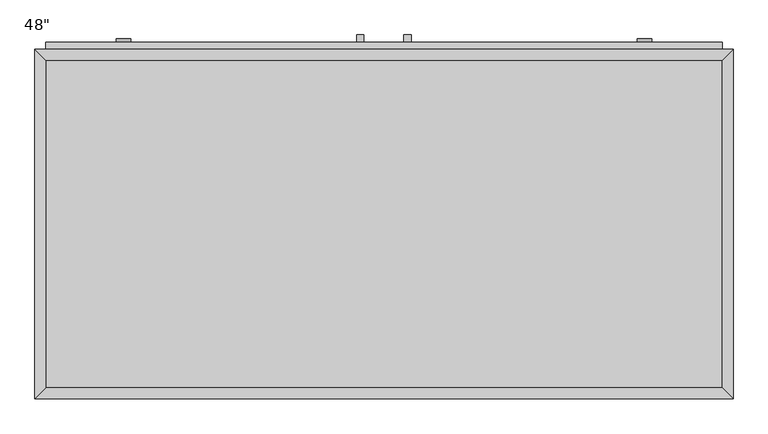
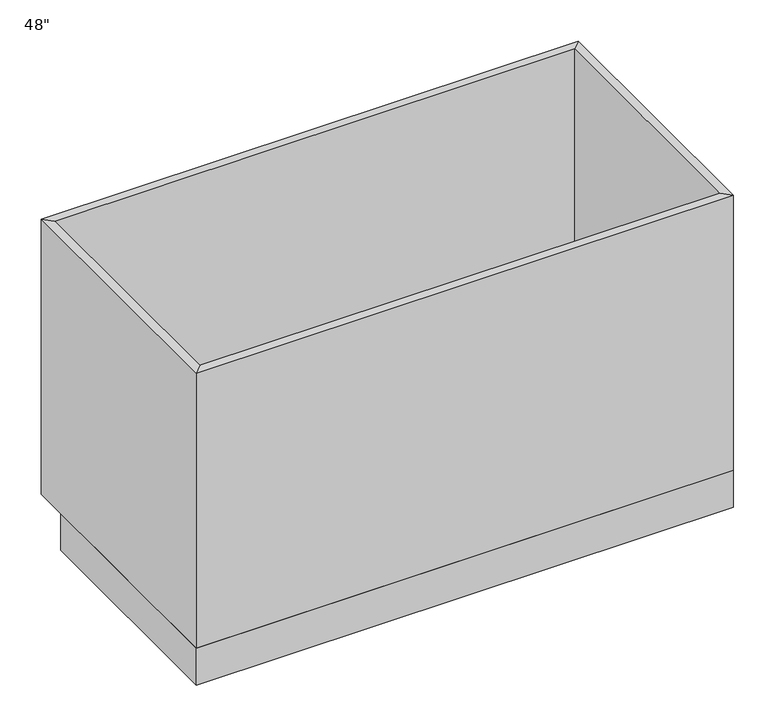
"""IFC4 building model written with IfcOpenShell, lengths in millimetres: furniture geometry."""

import ifcopenshell
import ifcopenshell.guid

model = None  # the IFC model being written
_history = None  # IfcOwnerHistory: only IFC2X3 demands one
_inside = {}  # id of a spatial element -> (the spatial element, [elements in it])
_under = {}  # id of a project, library or spatial element -> (it, [spatial elements below it])
_declared = {}  # id of a project -> (the project, [libraries it declares])
_typed = {}  # id of a type object -> (the type object, [elements of that type])
_made_of = {}  # id of a material, layer set ... -> (it, [elements and type objects made of it])


def new_model(schema):
    """Start an empty IFC model of exactly this schema.

    Asked for "IFC4X3", IfcOpenShell would pick the latest addendum, in which some entities
    have other attributes; the version numbers below select the first issue.
    IFC2X3 requires an IfcOwnerHistory on every rooted entity: one is made here for all.
    """
    global model, _history
    if schema == "IFC4X3":
        model = ifcopenshell.file(schema_version=(4, 3, 0, 0))
    else:
        model = ifcopenshell.file(schema=schema)
    _inside.clear()
    _under.clear()
    _declared.clear()
    _typed.clear()
    _made_of.clear()
    _history = None
    if model.schema == "IFC2X3":
        org = make("IfcOrganization", Name="unknown")
        user = make(
            "IfcPersonAndOrganization",
            ThePerson=make("IfcPerson", FamilyName="unknown"),
            TheOrganization=org,
        )
        app = make(
            "IfcApplication",
            ApplicationDeveloper=org,
            Version="unknown",
            ApplicationFullName="unknown",
            ApplicationIdentifier="unknown",
        )
        _history = make(
            "IfcOwnerHistory",
            OwningUser=user,
            OwningApplication=app,
            ChangeAction="ADDED",
            CreationDate=0,
        )
    return model


def make(cls, **values):
    """One entity of the class cls with the attributes given. An attribute that is None is left unset."""
    return model.create_entity(
        cls, **{name: value for name, value in values.items() if value is not None}
    )


def rooted(cls, **values):
    """An entity with a GlobalId (a new one), such as an element, a storey or a relation."""
    return make(cls, GlobalId=ifcopenshell.guid.new(), OwnerHistory=_history, **values)


def si_unit(unit_type, name, prefix=None):
    """IfcSIUnit, for example si_unit("LENGTHUNIT", "METRE", prefix="MILLI")."""
    return make("IfcSIUnit", UnitType=unit_type, Prefix=prefix, Name=name)


def assignment(units):
    """IfcUnitAssignment: the units of a project."""
    return None if units is None else make("IfcUnitAssignment", Units=units)


def point(xyz):
    """IfcCartesianPoint."""
    return None if xyz is None else make("IfcCartesianPoint", Coordinates=xyz)


def direction(xyz):
    """IfcDirection."""
    return None if xyz is None else make("IfcDirection", DirectionRatios=xyz)


def frame(location, z_axis=None, x_axis=None):
    """IfcAxis2Placement3D, a coordinate frame: its origin and axes. An axis left out is left unset."""
    return make(
        "IfcAxis2Placement3D",
        Location=point(location),
        Axis=direction(z_axis),
        RefDirection=direction(x_axis),
    )


def frame_2d(location, x_axis=None):
    """IfcAxis2Placement2D, a coordinate frame in the plane: its origin and x axis."""
    return make(
        "IfcAxis2Placement2D", Location=point(location), RefDirection=direction(x_axis)
    )


def origin():
    """The frame at (0, 0, 0) with its axes left unset."""
    return frame((0.0, 0.0, 0.0))


def origin_with_axes():
    """The frame at (0, 0, 0) with the z axis (0, 0, 1) and the x axis (1, 0, 0) written out."""
    return frame((0.0, 0.0, 0.0), z_axis=(0.0, 0.0, 1.0), x_axis=(1.0, 0.0, 0.0))


def place(relative_to, where):
    """IfcLocalPlacement: puts the frame where relative to a parent placement (None: the world)."""
    return make(
        "IfcLocalPlacement", PlacementRelTo=relative_to, RelativePlacement=where
    )


def context(
    kind, dimensions, precision=None, world=None, true_north=None, identifier=None
):
    """IfcGeometricRepresentationContext, for example the 3D "Model" context."""
    return make(
        "IfcGeometricRepresentationContext",
        ContextIdentifier=identifier,
        ContextType=kind,
        CoordinateSpaceDimension=dimensions,
        Precision=precision,
        WorldCoordinateSystem=world,
        TrueNorth=true_north,
    )


def project(units=None, contexts=None):
    """IfcProject with its units and contexts."""
    return rooted(
        "IfcProject",
        Name="project",
        RepresentationContexts=contexts,
        UnitsInContext=assignment(units),
    )


def spatial(cls, under=None, at=None, **own):
    """A site, building, storey or space (cls), placed at a placement, below another one or the project."""
    s = rooted(cls, ObjectPlacement=at, **own)
    if under is not None:
        _under.setdefault(under.id(), (under, []))[1].append(s)
    return s


def polyline(points):
    """IfcPolyline through the points."""
    return make("IfcPolyline", Points=[point(p) for p in points])


def circle_curve(where, radius):
    """IfcCircle in the frame where."""
    return make("IfcCircle", Position=where, Radius=radius)


def trimmed(basis, trim1, trim2, sense, master):
    """IfcTrimmedCurve: the piece of a basis curve between two trims."""
    return make(
        "IfcTrimmedCurve",
        BasisCurve=basis,
        Trim1=trim1,
        Trim2=trim2,
        SenseAgreement=sense,
        MasterRepresentation=master,
    )


def segment(curve, same_sense, transition):
    """IfcCompositeCurveSegment."""
    return make(
        "IfcCompositeCurveSegment",
        Transition=transition,
        SameSense=same_sense,
        ParentCurve=curve,
    )


def composite_curve(segments, self_intersect=None):
    """IfcCompositeCurve: segments joined end to end."""
    return make("IfcCompositeCurve", Segments=segments, SelfIntersect=self_intersect)


def outline(outer, holes=None, kind="AREA"):
    """IfcArbitraryClosedProfileDef: a profile drawn as a closed curve; with holes, ...WithVoids."""
    if holes is None:
        return make("IfcArbitraryClosedProfileDef", ProfileType=kind, OuterCurve=outer)
    return make(
        "IfcArbitraryProfileDefWithVoids",
        ProfileType=kind,
        OuterCurve=outer,
        InnerCurves=holes,
    )


def extrude(swept, where, along, depth):
    """IfcExtrudedAreaSolid: the profile swept, set in the frame where, extruded along a direction by depth."""
    return make(
        "IfcExtrudedAreaSolid",
        SweptArea=swept,
        Position=where,
        ExtrudedDirection=direction(along),
        Depth=depth,
    )


def faces_of(points, faces, orient=None, outer=None):
    """IfcFace entities. A face is a list of loops; a loop is a list of indices into points, from 0.

    orient and outer hold one flag for each loop. By default every Orientation is true, the
    first loop of a face is its IfcFaceOuterBound and the others are IfcFaceBound.
    """
    made = []
    for i, loops in enumerate(faces):
        bounds = []
        for j, loop in enumerate(loops):
            is_outer = j == 0 if outer is None else outer[i][j]
            bounds.append(
                make(
                    "IfcFaceOuterBound" if is_outer else "IfcFaceBound",
                    Bound=make("IfcPolyLoop", Polygon=[points[k] for k in loop]),
                    Orientation=True if orient is None else orient[i][j],
                )
            )
        made.append(make("IfcFace", Bounds=bounds))
    return made


def faceted_brep(points, faces, orient=None, outer=None, voids=None):
    """IfcFacetedBrep: a solid bounded by flat faces; with voids (closed shells), ...WithVoids."""
    shared = [point(p) for p in points]
    hull = make("IfcClosedShell", CfsFaces=faces_of(shared, faces, orient, outer))
    if voids is None:
        return make("IfcFacetedBrep", Outer=hull)
    return make(
        "IfcFacetedBrepWithVoids",
        Outer=hull,
        Voids=[
            make(cls, CfsFaces=faces_of(shared, fs, o, b)) for cls, fs, o, b in voids
        ],
    )


def shape(context_of_items, identifier, shape_type, items):
    """IfcShapeRepresentation: the items that make up one representation, for example the "Body"."""
    return make(
        "IfcShapeRepresentation",
        ContextOfItems=context_of_items,
        RepresentationIdentifier=identifier,
        RepresentationType=shape_type,
        Items=items,
    )


def source(mapping_origin, context_of_items, identifier, shape_type, items):
    """IfcRepresentationMap: a shape defined once, which mapped items show again and again."""
    return make(
        "IfcRepresentationMap",
        MappingOrigin=mapping_origin,
        MappedRepresentation=shape(context_of_items, identifier, shape_type, items),
    )


def transform(
    local_origin,
    x_axis=None,
    y_axis=None,
    z_axis=None,
    scale=None,
    scale2=None,
    scale3=None,
    uniform=True,
):
    """IfcCartesianTransformationOperator3D, or its non-uniform kind. x_axis, y_axis, z_axis: its Axis1, 2, 3."""
    if uniform:
        return make(
            "IfcCartesianTransformationOperator3D",
            Axis1=direction(x_axis),
            Axis2=direction(y_axis),
            LocalOrigin=point(local_origin),
            Scale=scale,
            Axis3=direction(z_axis),
        )
    return make(
        "IfcCartesianTransformationOperator3DnonUniform",
        Axis1=direction(x_axis),
        Axis2=direction(y_axis),
        LocalOrigin=point(local_origin),
        Scale=scale,
        Axis3=direction(z_axis),
        Scale2=scale2,
        Scale3=scale3,
    )


def mapped(mapping_source, mapping_target):
    """IfcMappedItem: shows the shape of a source again, moved by a transform."""
    return make(
        "IfcMappedItem", MappingSource=mapping_source, MappingTarget=mapping_target
    )


def made_of(thing, what):
    """Note that an element or type object is made of a material, layer set ...; save() writes the relation."""
    if what is not None:
        _made_of.setdefault(what.id(), (what, []))[1].append(thing)
    return thing


def element(
    cls,
    number,
    at=None,
    inside=None,
    cuts=None,
    type_object=None,
    material=None,
    context=None,
    identifier="Body",
    shape_type=None,
    held_by="IfcProductDefinitionShape",
    body=None,
    shapes=None,
    **own,
):
    """One element of the class cls, such as IfcWall. Its Tag is "e" and its number.

    at: its placement. inside: the storey or other place that contains it. cuts: it is an
    opening in that element (IfcRelVoidsElement). A single representation is given by context,
    identifier, shape_type and body (its items); several are given by shapes. held_by: the class
    of the entity that holds the representations. save() writes the other relations.
    """
    e = rooted(cls, Tag="e%d" % number, ObjectPlacement=at, **own)
    if body is not None:
        shapes = [shape(context, identifier, shape_type, body)]
    if shapes is not None:
        e.Representation = make(held_by, Representations=shapes)
    if inside is not None:
        _inside.setdefault(inside.id(), (inside, []))[1].append(e)
    if cuts is not None:
        rooted(
            "IfcRelVoidsElement", RelatingBuildingElement=cuts, RelatedOpeningElement=e
        )
    if type_object is not None:
        _typed.setdefault(type_object.id(), (type_object, []))[1].append(e)
    return made_of(e, material)


def aggregate(whole, parts):
    """IfcRelAggregates: a whole, such as a stair, and the parts it consists of."""
    return rooted("IfcRelAggregates", RelatingObject=whole, RelatedObjects=parts)


def save(model, path):
    """Write the relations noted so far, then the file.

    IfcRelAggregates (storeys below a building ...), IfcRelContainedInSpatialStructure (elements
    in a storey), IfcRelDefinesByType, IfcRelAssociatesMaterial and IfcRelDeclares: one each for
    every whole, place, type object, material and project.
    """
    for whole, parts in _under.values():
        aggregate(whole, parts)
    for where, things in _inside.values():
        rooted(
            "IfcRelContainedInSpatialStructure",
            RelatedElements=things,
            RelatingStructure=where,
        )
    for kind, things in _typed.values():
        rooted("IfcRelDefinesByType", RelatedObjects=things, RelatingType=kind)
    for what, things in _made_of.values():
        rooted("IfcRelAssociatesMaterial", RelatedObjects=things, RelatingMaterial=what)
    for by, libraries in _declared.values():
        rooted("IfcRelDeclares", RelatingContext=by, RelatedDefinitions=libraries)
    model.write(path)


def furniture_1910af95(model_context):
    return source(origin(), model_context, "Body", "SolidModel", [
        extrude(outline(polyline([(55.91996, 635.0), (55.91996, 622.3), (43.21996, 622.3), (43.21996, 635.0), (55.91996, 635.0)])), frame((0.0, 0.0, 469.9), z_axis=(0.0, 0.0, 1.0), x_axis=(1.0, 0.0, 0.0)), (0.0, 0.0, 1.0), 101.6),
        extrude(outline(polyline([(138.46996, 635.0), (138.46996, 622.3), (125.76996, 622.3), (125.76996, 635.0), (138.46996, 635.0)])), frame((0.0, 0.0, 469.9), z_axis=(0.0, 0.0, 1.0), x_axis=(1.0, 0.0, 0.0)), (0.0, 0.0, 1.0), 101.6),
        extrude(outline(composite_curve([segment(trimmed(circle_curve(frame_2d((484.1875, -363.97379)), 12.7), [point((484.1875, -376.67379))], [point((484.1875, -351.27379))], False, "CARTESIAN"), True, "CONTINUOUS"), segment(trimmed(circle_curve(frame_2d((484.1875, -363.97379)), 12.7), [point((484.1875, -351.27379))], [point((484.1875, -376.67379))], False, "CARTESIAN"), True, "CONTINUOUS")], self_intersect=False)), frame((0.0, 622.3, 0.0), z_axis=(0.0, 1.0, 0.0), x_axis=(0.0, 0.0, 1.0)), (0.0, 0.0, 1.0), 6.35),
        extrude(outline(composite_curve([segment(trimmed(circle_curve(frame_2d((233.3625, -363.97379)), 12.7), [point((233.3625, -376.67379))], [point((233.3625, -351.27379))], False, "CARTESIAN"), True, "CONTINUOUS"), segment(trimmed(circle_curve(frame_2d((233.3625, -363.97379)), 12.7), [point((233.3625, -351.27379))], [point((233.3625, -376.67379))], False, "CARTESIAN"), True, "CONTINUOUS")], self_intersect=False)), frame((0.0, 622.3, 0.0), z_axis=(0.0, 1.0, 0.0), x_axis=(0.0, 0.0, 1.0)), (0.0, 0.0, 1.0), 6.35),
        extrude(outline(composite_curve([segment(trimmed(circle_curve(frame_2d((233.3625, 545.66371)), 12.7), [point((233.3625, 532.96371))], [point((233.3625, 558.36371))], False, "CARTESIAN"), True, "CONTINUOUS"), segment(trimmed(circle_curve(frame_2d((233.3625, 545.66371)), 12.7), [point((233.3625, 558.36371))], [point((233.3625, 532.96371))], False, "CARTESIAN"), True, "CONTINUOUS")], self_intersect=False)), frame((0.0, 622.3, 0.0), z_axis=(0.0, 1.0, 0.0), x_axis=(0.0, 0.0, 1.0)), (0.0, 0.0, 1.0), 6.35),
        extrude(outline(composite_curve([segment(trimmed(circle_curve(frame_2d((484.1875, 545.66371)), 12.7), [point((484.1875, 532.96371))], [point((484.1875, 558.36371))], False, "CARTESIAN"), True, "CONTINUOUS"), segment(trimmed(circle_curve(frame_2d((484.1875, 545.66371)), 12.7), [point((484.1875, 558.36371))], [point((484.1875, 532.96371))], False, "CARTESIAN"), True, "CONTINUOUS")], self_intersect=False)), frame((0.0, 622.3, 0.0), z_axis=(0.0, 1.0, 0.0), x_axis=(0.0, 0.0, 1.0)), (0.0, 0.0, 1.0), 6.35),
        extrude(outline(polyline([(681.39496, 19.05), (-499.70504, 19.05), (-499.70504, 590.55), (681.39496, 590.55), (681.39496, 19.05)])), frame((0.0, 0.0, 88.9), z_axis=(0.0, 0.0, 1.0), x_axis=(1.0, 0.0, 0.0)), (0.0, 0.0, 1.0), 19.05),
        faceted_brep([(681.39496, 590.55, 749.3), (-499.70504, 590.55, 749.3), (-499.70504, 590.55, 88.9), (681.39496, 590.55, 88.9), (700.44496, 609.6, 749.3), (-518.75504, 609.6, 749.3), (700.44496, 609.6, 88.9), (-518.75504, 609.6, 88.9), (-499.70504, 19.05, 749.3), (-499.70504, 19.05, 88.9), (-518.75504, 0.0, 749.3), (-518.75504, 0.0, 88.9), (681.39496, 19.05, 749.3), (681.39496, 19.05, 88.9), (700.44496, 0.0, 749.3), (700.44496, 0.0, 88.9)], [[[0, 1, 2, 3]], [[4, 5, 1, 0]], [[6, 7, 5, 4]], [[3, 2, 7, 6]], [[1, 8, 9, 2]], [[5, 10, 8, 1]], [[7, 11, 10, 5]], [[2, 9, 11, 7]], [[8, 12, 13, 9]], [[10, 14, 12, 8]], [[11, 15, 14, 10]], [[9, 13, 15, 11]], [[12, 0, 3, 13]], [[14, 4, 0, 12]], [[15, 6, 4, 14]], [[13, 3, 6, 15]]]),
        extrude(outline(polyline([(700.44496, 0.0), (-518.75504, 0.0), (-518.75504, 533.4), (700.44496, 533.4), (700.44496, 0.0)])), origin_with_axes(), (0.0, 0.0, 1.0), 88.9),
        extrude(outline(polyline([(681.39496, 622.3), (681.39496, 609.6), (-499.70504, 609.6), (-499.70504, 622.3), (681.39496, 622.3)])), frame((0.0, 0.0, 628.65), z_axis=(0.0, 0.0, 1.0), x_axis=(1.0, 0.0, 0.0)), (0.0, 0.0, 1.0), 101.6),
        extrude(outline(polyline([(681.39496, 622.3), (681.39496, 609.6), (409.93246, 609.6), (409.93246, 622.3), (681.39496, 622.3)])), frame((0.0, 0.0, 361.95), z_axis=(0.0, 0.0, 1.0), x_axis=(1.0, 0.0, 0.0)), (0.0, 0.0, 1.0), 247.65),
        extrude(outline(polyline([(681.39496, 622.3), (681.39496, 609.6), (409.93246, 609.6), (409.93246, 622.3), (681.39496, 622.3)])), frame((0.0, 0.0, 107.95), z_axis=(0.0, 0.0, 1.0), x_axis=(1.0, 0.0, 0.0)), (0.0, 0.0, 1.0), 247.65),
        extrude(outline(polyline([(-228.24254, 622.3), (-228.24254, 609.6), (-499.70504, 609.6), (-499.70504, 622.3), (-228.24254, 622.3)])), frame((0.0, 0.0, 361.95), z_axis=(0.0, 0.0, 1.0), x_axis=(1.0, 0.0, 0.0)), (0.0, 0.0, 1.0), 247.65),
        extrude(outline(polyline([(-228.24254, 622.3), (-228.24254, 609.6), (-499.70504, 609.6), (-499.70504, 622.3), (-228.24254, 622.3)])), frame((0.0, 0.0, 107.95), z_axis=(0.0, 0.0, 1.0), x_axis=(1.0, 0.0, 0.0)), (0.0, 0.0, 1.0), 247.65),
        extrude(outline(polyline([(81.31996, 622.3), (81.31996, 609.6), (-209.19254, 609.6), (-209.19254, 622.3), (81.31996, 622.3)])), frame((0.0, 0.0, 107.95), z_axis=(0.0, 0.0, 1.0), x_axis=(1.0, 0.0, 0.0)), (0.0, 0.0, 1.0), 501.65),
        extrude(outline(polyline([(390.88246, 622.3), (390.88246, 609.6), (100.36996, 609.6), (100.36996, 622.3), (390.88246, 622.3)])), frame((0.0, 0.0, 107.95), z_axis=(0.0, 0.0, 1.0), x_axis=(1.0, 0.0, 0.0)), (0.0, 0.0, 1.0), 501.65),
    ])


if __name__ == "__main__":
    model = new_model("IFC4")
    model_context = context("Model", 3, world=origin())
    ifc_project = project(units=[si_unit("LENGTHUNIT", "METRE", prefix="MILLI")], contexts=[model_context])
    site = spatial("IfcSite", under=ifc_project)
    building = spatial("IfcBuilding", under=site)
    placement = place(None, origin())
    furniture_shape = furniture_1910af95(model_context)
    element("IfcFurniture", 1, ObjectType="Vanity Cabinet-Double Door & 4 Drawer : 48\"", at=placement, inside=building, context=model_context, shape_type="MappedRepresentation", body=[
        mapped(furniture_shape, transform((0.0, 0.0, 0.0), x_axis=(1.0, 0.0, 0.0), y_axis=(0.0, 1.0, 0.0), z_axis=(0.0, 0.0, 1.0))),
    ])
    save(model, "model.ifc")

# Revit data of these elements
# Type "Vanity Cabinet-Double Door & 4 Drawer : 48\""
#   Assembly Code = "C1030410"
#   Depth = 2' - 0"
#   Height = 2' - 5 1/2"
#   Toe Depth = 0' - 3"
#   Toe Height = 0' - 3 1/2"
#   Width = 4' - 0"
#   Cabinet Material = Cherry
#   Door/Drawer Material = Cherry
#   Handle Material = Steel, Chrome Plated
#   Default Elevation = 0
# Element 1 (IfcFurniture, "Vanity Cabinet-Double Door & 4 Drawer : 48\"")
#   Materials on its faces: "Cherry", "Steel, Chrome Plated", "Cabinets"
# Materials
#   "Cherry": class "Wood", colour RGB 157 77 38, transparency 0, Description = "Prunus Serotina", Cost = 0
#   "Steel, Chrome Plated": class "Metal", colour RGB 120 120 120, transparency 0, Description = "Chromiuim plated steel", Cost = 0
#   "Cabinets": class "Unassigned", colour RGB 249 249 249, transparency 0
